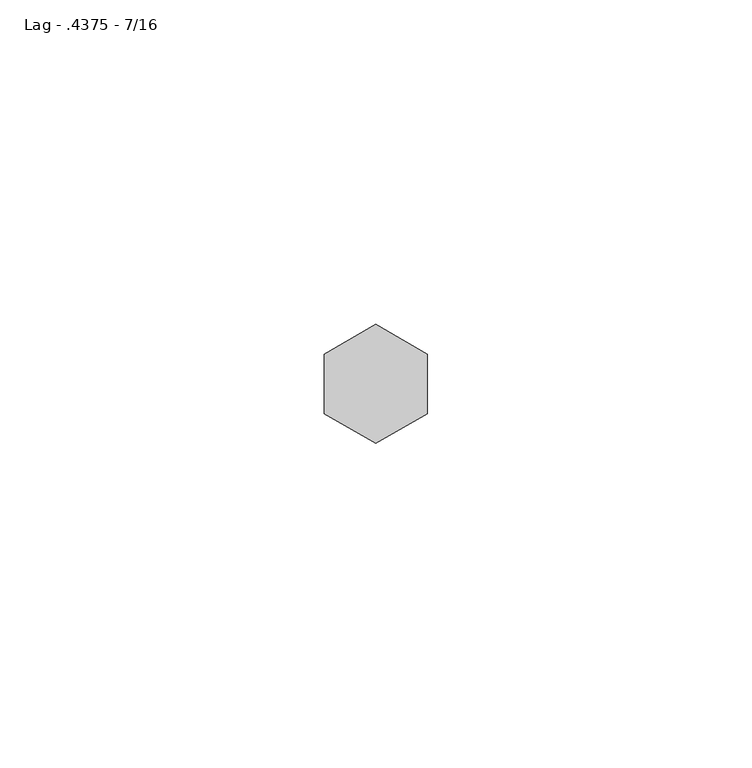
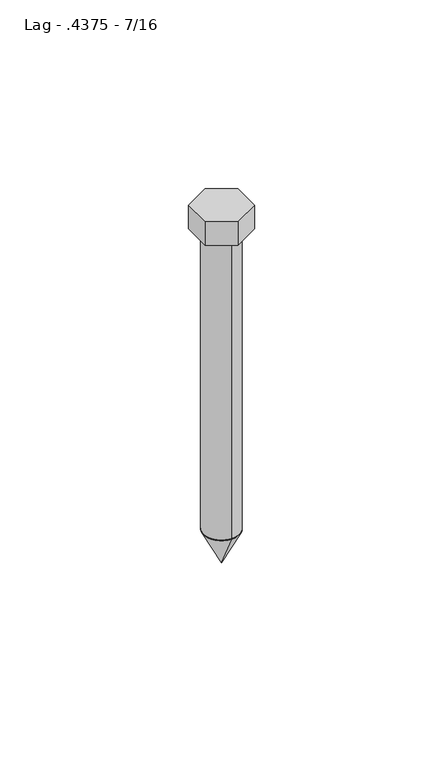
"""IFC4 building model written with IfcOpenShell, lengths in millimetres: fastener geometry, 060523 - W_P_C - Fastenings - Generic : Lag - .4375 - 7/16."""

from ifc_helpers import new_model, si_unit, point, frame, origin, origin_with_axes, origin_2d, place, context, project, spatial, polyline, circle_curve, trimmed, segment, composite_curve, outline, extrude, source, transform, mapped, element, save
from ifc_brep_helpers import plane_surface, revolved_surface, advanced_brep


def lag_4375_7_16_73db41da(model_context):
    return source(origin(), model_context, "Body", "SolidModel", [
        advanced_brep(
        [(0.0, -5.7546875, -101.6), (0.0, 5.7546875, -101.6), (0.0, 0.0, -101.6), (0.0, 0.0, -113.109375)],
        [
            (0, 1, circle_curve(frame((0.0, 0.0, -101.6), z_axis=(0.0, 0.0, 1.0), x_axis=(0.0, 1.0, 0.0)), 5.7546875)),
            (1, 2),
            (2, 0),
            (1, 0, circle_curve(frame((0.0, 0.0, -101.6), z_axis=(0.0, 0.0, 1.0), x_axis=(0.0, 1.0, 0.0)), 5.7546875)),
            (3, 1),
            (0, 3),
        ],
        [
            plane_surface(frame((0.0, 0.0, -101.6), z_axis=(0.0, 0.0, 1.0), x_axis=(0.0, 1.0, 0.0))),
            revolved_surface(polyline([(0.0, 5.7546875, -101.6), (0.0, 0.0, -113.109375)]), (0.0, 0.0, -103.0840259), (0.0, 0.0, -1.0)),
        ],
        [
            (0, [[1, 2, 3]]),
            (0, [[4, -3, -2]]),
            (1, [[5, -1, 6]]),
            (1, [[-6, -4, -5]]),
        ],
    ),
        extrude(outline(polyline([(-7.9375, 4.5827178), (0.0, 9.1654355), (7.9375, 4.5827178), (7.9375, -4.5827178), (0.0, -9.1654355), (-7.9375, -4.5827178), (-7.9375, 4.5827178)])), origin_with_axes(), (0.0, 0.0, 1.0), 8.0367187),
        extrude(outline(composite_curve([segment(trimmed(circle_curve(origin_2d(), 5.7546875), [point((0.0, -5.7546875))], [point((0.0, 5.7546875))], False, "CARTESIAN"), True, "CONTINUOUS"), segment(trimmed(circle_curve(origin_2d(), 5.7546875), [point((0.0, 5.7546875))], [point((0.0, -5.7546875))], False, "CARTESIAN"), True, "CONTINUOUS")], self_intersect=False)), frame((0.0, 0.0, -101.6), z_axis=(0.0, 0.0, 1.0), x_axis=(1.0, 0.0, 0.0)), (0.0, 0.0, 1.0), 101.6),
    ])


if __name__ == "__main__":
    model = new_model("IFC4")
    model_context = context("Model", 3, world=origin())
    ifc_project = project(units=[si_unit("LENGTHUNIT", "METRE", prefix="MILLI")], contexts=[model_context])
    site = spatial("IfcSite", under=ifc_project)
    building = spatial("IfcBuilding", under=site)
    placement = place(None, origin())
    lag_4375_7_16_shape = lag_4375_7_16_73db41da(model_context)
    element("IfcFastener", 1, ObjectType="060523 - W_P_C - Fastenings - Generic : Lag - .4375 - 7/16", at=placement, inside=building, context=model_context, shape_type="MappedRepresentation", body=[
        mapped(lag_4375_7_16_shape, transform((0.0, 0.0, 0.0), x_axis=(1.0, 0.0, 0.0), y_axis=(0.0, 1.0, 0.0), z_axis=(0.0, 0.0, 1.0))),
    ])
    save(model, "model.ifc")

# Revit data of these elements
# Type "060523 - W_P_C - Fastenings - Generic : Lag - .4375 - 7/16"
#   Washer_Thickness = 0' - 0 27/256"
#   Washer Radius = 0' - 0 139/256"
#   Washer Offset - Head = 0' - 0"
#   Washer Offset = 0' - 0"
#   Thickness_of_Substrate [instance default] = 0' - 1"
#   Side = 0' - 0.36133"
#   Radius = 0' - 0 29/128"
#   Length [instance default] = 0' - 4"
#   Head Size = 0' - 0 5/8"
#   Head Radius = 0' - 0 5/16"
#   Head Height = 0' - 0 81/256"
#   Double Diameter = 0' - 0 29/32"
#   Diameter = 0' - 0 29/64"
#   Default Elevation = 4' - 0"
#   Washer_Nut_Visibility = no
#   Washer_Head_Visibility = no
#   Round_Head_Visibility = no
#   Point Visibility = yes
#   Nut_Visibility = no
#   Hex_Head_Visiblilty = yes
#   Washer Material = none
#   Bolt Material (Size) = AT SILL - FASTENER AT 24" O.C.
# Element 1 (IfcFastener, "060523 - W_P_C - Fastenings - Generic : Lag - .4375 - 7/16")
#   Materials on its faces: "AT SILL - FASTENER AT 24\" O.C."
# Materials
#   "AT SILL - FASTENER AT 24\" O.C.": class "Generic", colour RGB 120 120 120, transparency 0, Cost = 0
